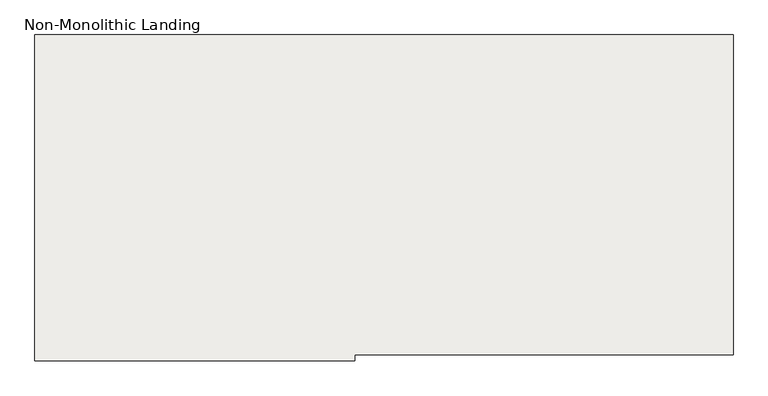
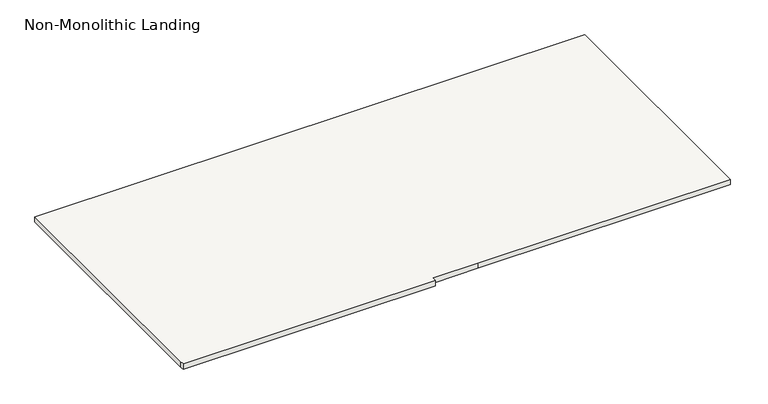
"""IFC4 building model written with IfcOpenShell, lengths in millimetres: slab geometry, Non-Monolithic Landing."""

import ifcopenshell
import ifcopenshell.guid

model = None  # the IFC model being written
_history = None  # IfcOwnerHistory: only IFC2X3 demands one
_inside = {}  # id of a spatial element -> (the spatial element, [elements in it])
_under = {}  # id of a project, library or spatial element -> (it, [spatial elements below it])
_declared = {}  # id of a project -> (the project, [libraries it declares])
_typed = {}  # id of a type object -> (the type object, [elements of that type])
_made_of = {}  # id of a material, layer set ... -> (it, [elements and type objects made of it])


def new_model(schema):
    """Start an empty IFC model of exactly this schema.

    Asked for "IFC4X3", IfcOpenShell would pick the latest addendum, in which some entities
    have other attributes; the version numbers below select the first issue.
    IFC2X3 requires an IfcOwnerHistory on every rooted entity: one is made here for all.
    """
    global model, _history
    if schema == "IFC4X3":
        model = ifcopenshell.file(schema_version=(4, 3, 0, 0))
    else:
        model = ifcopenshell.file(schema=schema)
    _inside.clear()
    _under.clear()
    _declared.clear()
    _typed.clear()
    _made_of.clear()
    _history = None
    if model.schema == "IFC2X3":
        org = make("IfcOrganization", Name="unknown")
        user = make(
            "IfcPersonAndOrganization",
            ThePerson=make("IfcPerson", FamilyName="unknown"),
            TheOrganization=org,
        )
        app = make(
            "IfcApplication",
            ApplicationDeveloper=org,
            Version="unknown",
            ApplicationFullName="unknown",
            ApplicationIdentifier="unknown",
        )
        _history = make(
            "IfcOwnerHistory",
            OwningUser=user,
            OwningApplication=app,
            ChangeAction="ADDED",
            CreationDate=0,
        )
    return model


def make(cls, **values):
    """One entity of the class cls with the attributes given. An attribute that is None is left unset."""
    return model.create_entity(
        cls, **{name: value for name, value in values.items() if value is not None}
    )


def rooted(cls, **values):
    """An entity with a GlobalId (a new one), such as an element, a storey or a relation."""
    return make(cls, GlobalId=ifcopenshell.guid.new(), OwnerHistory=_history, **values)


def si_unit(unit_type, name, prefix=None):
    """IfcSIUnit, for example si_unit("LENGTHUNIT", "METRE", prefix="MILLI")."""
    return make("IfcSIUnit", UnitType=unit_type, Prefix=prefix, Name=name)


def assignment(units):
    """IfcUnitAssignment: the units of a project."""
    return None if units is None else make("IfcUnitAssignment", Units=units)


def point(xyz):
    """IfcCartesianPoint."""
    return None if xyz is None else make("IfcCartesianPoint", Coordinates=xyz)


def direction(xyz):
    """IfcDirection."""
    return None if xyz is None else make("IfcDirection", DirectionRatios=xyz)


def frame(location, z_axis=None, x_axis=None):
    """IfcAxis2Placement3D, a coordinate frame: its origin and axes. An axis left out is left unset."""
    return make(
        "IfcAxis2Placement3D",
        Location=point(location),
        Axis=direction(z_axis),
        RefDirection=direction(x_axis),
    )


def origin():
    """The frame at (0, 0, 0) with its axes left unset."""
    return frame((0.0, 0.0, 0.0))


def place(relative_to, where):
    """IfcLocalPlacement: puts the frame where relative to a parent placement (None: the world)."""
    return make(
        "IfcLocalPlacement", PlacementRelTo=relative_to, RelativePlacement=where
    )


def context(
    kind, dimensions, precision=None, world=None, true_north=None, identifier=None
):
    """IfcGeometricRepresentationContext, for example the 3D "Model" context."""
    return make(
        "IfcGeometricRepresentationContext",
        ContextIdentifier=identifier,
        ContextType=kind,
        CoordinateSpaceDimension=dimensions,
        Precision=precision,
        WorldCoordinateSystem=world,
        TrueNorth=true_north,
    )


def project(units=None, contexts=None):
    """IfcProject with its units and contexts."""
    return rooted(
        "IfcProject",
        Name="project",
        RepresentationContexts=contexts,
        UnitsInContext=assignment(units),
    )


def spatial(cls, under=None, at=None, **own):
    """A site, building, storey or space (cls), placed at a placement, below another one or the project."""
    s = rooted(cls, ObjectPlacement=at, **own)
    if under is not None:
        _under.setdefault(under.id(), (under, []))[1].append(s)
    return s


def polyline(points):
    """IfcPolyline through the points."""
    return make("IfcPolyline", Points=[point(p) for p in points])


def outline(outer, holes=None, kind="AREA"):
    """IfcArbitraryClosedProfileDef: a profile drawn as a closed curve; with holes, ...WithVoids."""
    if holes is None:
        return make("IfcArbitraryClosedProfileDef", ProfileType=kind, OuterCurve=outer)
    return make(
        "IfcArbitraryProfileDefWithVoids",
        ProfileType=kind,
        OuterCurve=outer,
        InnerCurves=holes,
    )


def extrude(swept, where, along, depth):
    """IfcExtrudedAreaSolid: the profile swept, set in the frame where, extruded along a direction by depth."""
    return make(
        "IfcExtrudedAreaSolid",
        SweptArea=swept,
        Position=where,
        ExtrudedDirection=direction(along),
        Depth=depth,
    )


def shape(context_of_items, identifier, shape_type, items):
    """IfcShapeRepresentation: the items that make up one representation, for example the "Body"."""
    return make(
        "IfcShapeRepresentation",
        ContextOfItems=context_of_items,
        RepresentationIdentifier=identifier,
        RepresentationType=shape_type,
        Items=items,
    )


def source(mapping_origin, context_of_items, identifier, shape_type, items):
    """IfcRepresentationMap: a shape defined once, which mapped items show again and again."""
    return make(
        "IfcRepresentationMap",
        MappingOrigin=mapping_origin,
        MappedRepresentation=shape(context_of_items, identifier, shape_type, items),
    )


def transform(
    local_origin,
    x_axis=None,
    y_axis=None,
    z_axis=None,
    scale=None,
    scale2=None,
    scale3=None,
    uniform=True,
):
    """IfcCartesianTransformationOperator3D, or its non-uniform kind. x_axis, y_axis, z_axis: its Axis1, 2, 3."""
    if uniform:
        return make(
            "IfcCartesianTransformationOperator3D",
            Axis1=direction(x_axis),
            Axis2=direction(y_axis),
            LocalOrigin=point(local_origin),
            Scale=scale,
            Axis3=direction(z_axis),
        )
    return make(
        "IfcCartesianTransformationOperator3DnonUniform",
        Axis1=direction(x_axis),
        Axis2=direction(y_axis),
        LocalOrigin=point(local_origin),
        Scale=scale,
        Axis3=direction(z_axis),
        Scale2=scale2,
        Scale3=scale3,
    )


def mapped(mapping_source, mapping_target):
    """IfcMappedItem: shows the shape of a source again, moved by a transform."""
    return make(
        "IfcMappedItem", MappingSource=mapping_source, MappingTarget=mapping_target
    )


def made_of(thing, what):
    """Note that an element or type object is made of a material, layer set ...; save() writes the relation."""
    if what is not None:
        _made_of.setdefault(what.id(), (what, []))[1].append(thing)
    return thing


def element(
    cls,
    number,
    at=None,
    inside=None,
    cuts=None,
    type_object=None,
    material=None,
    context=None,
    identifier="Body",
    shape_type=None,
    held_by="IfcProductDefinitionShape",
    body=None,
    shapes=None,
    **own,
):
    """One element of the class cls, such as IfcWall. Its Tag is "e" and its number.

    at: its placement. inside: the storey or other place that contains it. cuts: it is an
    opening in that element (IfcRelVoidsElement). A single representation is given by context,
    identifier, shape_type and body (its items); several are given by shapes. held_by: the class
    of the entity that holds the representations. save() writes the other relations.
    """
    e = rooted(cls, Tag="e%d" % number, ObjectPlacement=at, **own)
    if body is not None:
        shapes = [shape(context, identifier, shape_type, body)]
    if shapes is not None:
        e.Representation = make(held_by, Representations=shapes)
    if inside is not None:
        _inside.setdefault(inside.id(), (inside, []))[1].append(e)
    if cuts is not None:
        rooted(
            "IfcRelVoidsElement", RelatingBuildingElement=cuts, RelatedOpeningElement=e
        )
    if type_object is not None:
        _typed.setdefault(type_object.id(), (type_object, []))[1].append(e)
    return made_of(e, material)


def aggregate(whole, parts):
    """IfcRelAggregates: a whole, such as a stair, and the parts it consists of."""
    return rooted("IfcRelAggregates", RelatingObject=whole, RelatedObjects=parts)


def save(model, path):
    """Write the relations noted so far, then the file.

    IfcRelAggregates (storeys below a building ...), IfcRelContainedInSpatialStructure (elements
    in a storey), IfcRelDefinesByType, IfcRelAssociatesMaterial and IfcRelDeclares: one each for
    every whole, place, type object, material and project.
    """
    for whole, parts in _under.values():
        aggregate(whole, parts)
    for where, things in _inside.values():
        rooted(
            "IfcRelContainedInSpatialStructure",
            RelatedElements=things,
            RelatingStructure=where,
        )
    for kind, things in _typed.values():
        rooted("IfcRelDefinesByType", RelatedObjects=things, RelatingType=kind)
    for what, things in _made_of.values():
        rooted("IfcRelAssociatesMaterial", RelatedObjects=things, RelatingMaterial=what)
    for by, libraries in _declared.values():
        rooted("IfcRelDeclares", RelatingContext=by, RelatedDefinitions=libraries)
    model.write(path)


def non_monolithic_landing_55c0a7d8(model_context):
    return source(origin(), model_context, "Body", "SweptSolid", [
        extrude(outline(polyline([(-22683.4414763, -9454.4070712), (-22877.1164763, -9454.4070712), (-22877.1164763, -9473.4570712), (-23943.9164763, -9473.4570712), (-23943.9164763, -9454.4070712), (-23943.9164763, -8387.6070712), (-21616.6414763, -8387.6070712), (-21616.6414763, -9454.4070712), (-22683.4414763, -9454.4070712)])), frame((0.0, 0.0, 1347.6882813), z_axis=(0.0, 0.0, 1.0), x_axis=(1.0, 0.0, 0.0)), (0.0, 0.0, 1.0), 23.9117188),
    ])


if __name__ == "__main__":
    model = new_model("IFC4")
    model_context = context("Model", 3, world=origin())
    ifc_project = project(units=[si_unit("LENGTHUNIT", "METRE", prefix="MILLI")], contexts=[model_context])
    site = spatial("IfcSite", under=ifc_project)
    building = spatial("IfcBuilding", under=site)
    placement = place(None, origin())
    non_monolithic_landing_shape = non_monolithic_landing_55c0a7d8(model_context)
    element("IfcSlab", 1, ObjectType="Non-Monolithic Landing", at=placement, inside=building, context=model_context, shape_type="MappedRepresentation", body=[
        mapped(non_monolithic_landing_shape, transform((0.0, 0.0, 0.0), x_axis=(1.0, 0.0, 0.0), y_axis=(0.0, 1.0, 0.0), z_axis=(0.0, 0.0, 1.0))),
    ])
    save(model, "model.ifc")

# Revit data of these elements
# Element 1 (IfcSlab, "Non-Monolithic Landing")
#   Materials on its faces: "Composite Deck - Trex - Select - 1x6 Square Edge Board - Saddle - 20'"
# Materials
#   "Composite Deck - Trex - Select - 1x6 Square Edge Board - Saddle - 20'": class "Wood", colour RGB 120 75 45, transparency 0, Keynote = "06 11 00", Model = "Trex Select® Composite Deck 1\" Square Edge Board", Manufacturer = "Trex", URL = "http://www.trex.com/", Description = "1x6 Trex Select® Composite Deck Square Edge Board", Cost = 0
